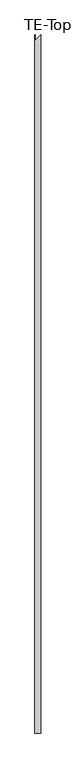
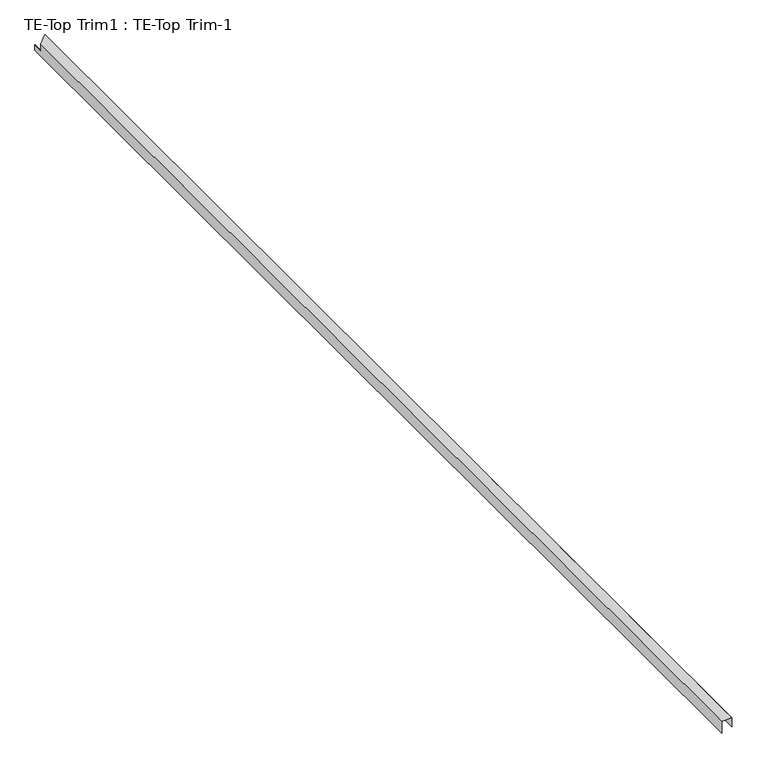
"""IFC4 building model written with IfcOpenShell, lengths in millimetres: proxy geometry, TE-Top Trim1 : TE-Top Trim-1."""

from ifc_helpers import new_model, si_unit, origin, place, context, project, spatial, faceted_brep, source, transform, mapped, element, save


def te_top_trim1_te_top_trim_1_5eaecf50(model_context):
    return source(origin(), model_context, "Body", "Brep", [
        faceted_brep([(590352.6755052, -531600.3289841, 2387.6), (590351.7825364, -531600.3289841, 2387.6), (590351.7825364, -531600.3289841, 2411.4125), (590352.6755052, -531600.3289841, 2411.4125), (590393.3931339, -531600.3289841, 2439.2929688), (590393.3931339, -531600.3289841, 2400.3), (590392.4558739, -531600.3289841, 2400.3), (590392.4558739, -531600.3289841, 2411.4125), (590392.4558739, -531600.3289841, 2438.4), (590392.4459322, -531600.3289841, 2439.2929688), (590352.6755052, -536420.7663841, 2387.6), (590352.6755052, -536420.7663841, 2438.4), (590392.4558739, -536420.7663841, 2438.4), (590392.4558739, -536420.7663841, 2400.3), (590393.3931339, -536420.7663841, 2400.3), (590393.3931339, -536420.7663841, 2439.2929688), (590351.7825364, -536420.7663841, 2439.2929688), (590351.7825364, -536420.7663841, 2387.6), (590351.7825364, -531640.9923799, 2439.2929688), (590351.7825364, -531640.9923799, 2411.4125), (590352.6755052, -531640.0994112, 2438.4), (590352.6755052, -531640.0994112, 2411.4125)], [[[0, 1, 2, 3]], [[4, 5, 6, 7, 8, 9]], [[10, 11, 12, 13, 14, 15, 16, 17]], [[1, 0, 10, 17]], [[17, 16, 18, 19, 2, 1]], [[16, 15, 4, 9, 18]], [[5, 4, 15, 14]], [[6, 5, 14, 13]], [[13, 12, 8, 7, 6]], [[12, 11, 20, 8]], [[11, 10, 0, 3, 21, 20]], [[19, 21, 3, 2]], [[21, 19, 18, 9, 8, 20]]]),
    ])


if __name__ == "__main__":
    model = new_model("IFC4")
    model_context = context("Model", 3, world=origin())
    ifc_project = project(units=[si_unit("LENGTHUNIT", "METRE", prefix="MILLI")], contexts=[model_context])
    site = spatial("IfcSite", under=ifc_project)
    building = spatial("IfcBuilding", under=site)
    placement = place(None, origin())
    te_top_trim1_te_top_trim_1_shape = te_top_trim1_te_top_trim_1_5eaecf50(model_context)
    element("IfcBuildingElementProxy", 1, Name="TE-Top Trim1 : TE-Top Trim-1", ObjectType="TE-Top Trim1 : TE-Top Trim-1", at=placement, inside=building, context=model_context, shape_type="MappedRepresentation", body=[
        mapped(te_top_trim1_te_top_trim_1_shape, transform((0.0, 0.0, 0.0), x_axis=(1.0, 0.0, 0.0), y_axis=(0.0, 1.0, 0.0), z_axis=(0.0, 0.0, 1.0))),
    ])
    save(model, "model.ifc")

# Revit data of these elements
# Element 1 (IfcBuildingElementProxy, "TE-Top Trim1 : TE-Top Trim-1")
#   Materials on its faces: "EDGE TRIM BY MTL PANEL MFR."
# Materials
#   "EDGE TRIM BY MTL PANEL MFR.": class "Generic", colour RGB 239 242 240, transparency 0, Cost = 0
